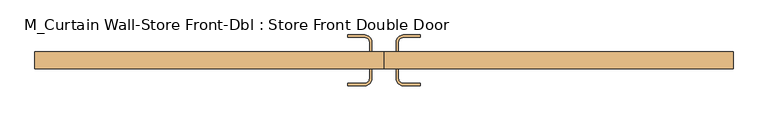
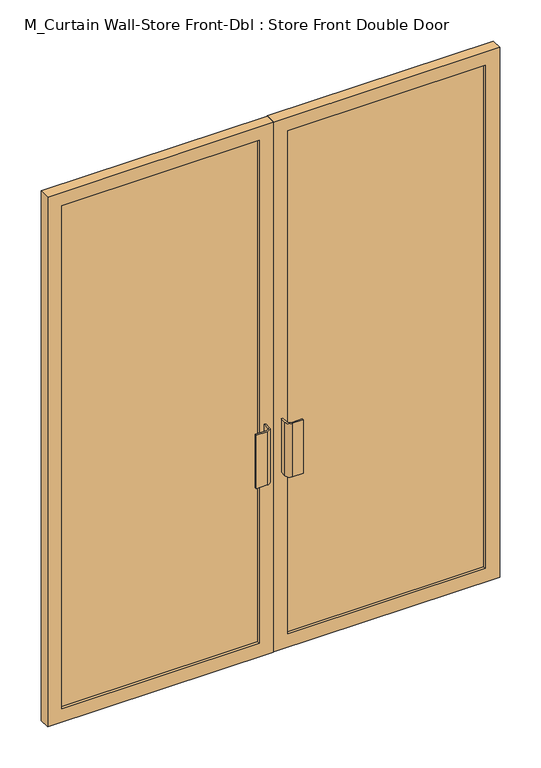
"""IFC4 building model written with IfcOpenShell, lengths in millimetres: door geometry, M_Curtain Wall-Store Front-Dbl : Store Front Double Door."""

from ifc_helpers import new_model, si_unit, point, frame, frame_2d, origin, place, context, project, spatial, polyline, circle_curve, trimmed, segment, composite_curve, outline, extrude, source, transform, mapped, element, save


def m_curtain_wall_store_front_dbl_store_front_double_door_46208f06(model_context):
    return source(origin(), model_context, "Body", "SweptSolid", [
        extrude(outline(composite_curve([segment(trimmed(circle_curve(frame_2d((-50.8, -14.85)), 19.05), [point((-31.75, -14.85))], [point((-50.8, -33.9))], False, "CARTESIAN"), True, "CONTINUOUS"), segment(polyline([(-50.8, -33.9), (-95.25, -33.9), (-95.25, -27.55), (-50.8, -27.55)]), True, "CONTINUOUS"), segment(trimmed(circle_curve(frame_2d((-50.8, -14.85)), 12.7), [point((-50.8, -27.55))], [point((-38.1, -14.85))], True, "CARTESIAN"), True, "CONTINUOUS"), segment(polyline([(-38.1, -14.85), (-38.1, 10.55), (-31.75, 10.55), (-31.75, -14.85)]), True, "CONTINUOUS")], self_intersect=False)), frame((0.0, 0.0, 762.0), z_axis=(0.0, 0.0, 1.0), x_axis=(1.0, 0.0, 0.0)), (0.0, 0.0, 1.0), 228.6),
        extrude(outline(composite_curve([segment(polyline([(31.75, -14.85), (31.75, 10.55), (38.1, 10.55), (38.1, -14.85)]), True, "CONTINUOUS"), segment(trimmed(circle_curve(frame_2d((50.8, -14.85)), 12.7), [point((38.1, -14.85))], [point((50.8, -27.55))], True, "CARTESIAN"), True, "CONTINUOUS"), segment(polyline([(50.8, -27.55), (95.25, -27.55), (95.25, -33.9), (50.8, -33.9)]), True, "CONTINUOUS"), segment(trimmed(circle_curve(frame_2d((50.8, -14.85)), 19.05), [point((50.8, -33.9))], [point((31.75, -14.85))], False, "CARTESIAN"), True, "CONTINUOUS")], self_intersect=False)), frame((0.0, 0.0, 762.0), z_axis=(0.0, 0.0, 1.0), x_axis=(1.0, 0.0, 0.0)), (0.0, 0.0, 1.0), 228.6),
        extrude(outline(composite_curve([segment(polyline([(-31.75, 80.4), (-31.75, 55.0), (-38.1, 55.0), (-38.1, 80.4)]), True, "CONTINUOUS"), segment(trimmed(circle_curve(frame_2d((-50.8, 80.4)), 12.7), [point((-38.1, 80.4))], [point((-50.8, 93.1))], True, "CARTESIAN"), True, "CONTINUOUS"), segment(polyline([(-50.8, 93.1), (-95.25, 93.1), (-95.25, 99.45), (-50.8, 99.45)]), True, "CONTINUOUS"), segment(trimmed(circle_curve(frame_2d((-50.8, 80.4)), 19.05), [point((-50.8, 99.45))], [point((-31.75, 80.4))], False, "CARTESIAN"), True, "CONTINUOUS")], self_intersect=False)), frame((0.0, 0.0, 762.0), z_axis=(0.0, 0.0, 1.0), x_axis=(1.0, 0.0, 0.0)), (0.0, 0.0, 1.0), 228.6),
        extrude(outline(composite_curve([segment(trimmed(circle_curve(frame_2d((50.8, 80.4)), 19.05), [point((31.75, 80.4))], [point((50.8, 99.45))], False, "CARTESIAN"), True, "CONTINUOUS"), segment(polyline([(50.8, 99.45), (95.25, 99.45), (95.25, 93.1), (50.8, 93.1)]), True, "CONTINUOUS"), segment(trimmed(circle_curve(frame_2d((50.8, 80.4)), 12.7), [point((50.8, 93.1))], [point((38.1, 80.4))], True, "CARTESIAN"), True, "CONTINUOUS"), segment(polyline([(38.1, 80.4), (38.1, 55.0), (31.75, 55.0), (31.75, 80.4)]), True, "CONTINUOUS")], self_intersect=False)), frame((0.0, 0.0, 762.0), z_axis=(0.0, 0.0, 1.0), x_axis=(1.0, 0.0, 0.0)), (0.0, 0.0, 1.0), 228.6),
        extrude(outline(polyline([(860.9333333, 23.25), (57.94375, 23.25), (57.94375, 42.3), (860.9333333, 42.3), (860.9333333, 23.25)])), frame((0.0, 0.0, 57.15), z_axis=(0.0, 0.0, 1.0), x_axis=(1.0, 0.0, 0.0)), (0.0, 0.0, 1.0), 2160.7),
        extrude(outline(polyline([(-57.94375, 23.25), (-860.9333333, 23.25), (-860.9333333, 42.3), (-57.94375, 42.3), (-57.94375, 23.25)])), frame((0.0, 0.0, 57.15), z_axis=(0.0, 0.0, 1.0), x_axis=(1.0, 0.0, 0.0)), (0.0, 0.0, 1.0), 2160.7),
        extrude(outline(polyline([(2275.0, 0.79375), (0.0, 0.79375), (0.0, 918.0833333), (2275.0, 918.0833333), (2275.0, 0.79375)]), holes=[polyline([(2217.85, 57.94375), (2217.85, 860.9333333), (57.15, 860.9333333), (57.15, 57.94375), (2217.85, 57.94375)])]), frame((0.0, 10.55, 0.0), z_axis=(0.0, 1.0, 0.0), x_axis=(0.0, 0.0, 1.0)), (0.0, 0.0, 1.0), 44.45),
        extrude(outline(polyline([(2275.0, -0.79375), (2275.0, -918.0833333), (0.0, -918.0833333), (0.0, -0.79375), (2275.0, -0.79375)]), holes=[polyline([(2217.85, -860.9333333), (2217.85, -57.94375), (57.15, -57.94375), (57.15, -860.9333333), (2217.85, -860.9333333)])]), frame((0.0, 10.55, 0.0), z_axis=(0.0, 1.0, 0.0), x_axis=(0.0, 0.0, 1.0)), (0.0, 0.0, 1.0), 44.45),
    ])


if __name__ == "__main__":
    model = new_model("IFC4")
    model_context = context("Model", 3, world=origin())
    ifc_project = project(units=[si_unit("LENGTHUNIT", "METRE", prefix="MILLI")], contexts=[model_context])
    site = spatial("IfcSite", under=ifc_project)
    building = spatial("IfcBuilding", under=site)
    placement = place(None, origin())
    m_curtain_wall_store_front_dbl_store_front_double_door_shape = m_curtain_wall_store_front_dbl_store_front_double_door_46208f06(model_context)
    element("IfcDoor", 1, ObjectType="M_Curtain Wall-Store Front-Dbl : Store Front Double Door", at=placement, inside=building, context=model_context, shape_type="MappedRepresentation", body=[
        mapped(m_curtain_wall_store_front_dbl_store_front_double_door_shape, transform((0.0, 0.0, 0.0), x_axis=(1.0, 0.0, 0.0), y_axis=(0.0, 1.0, 0.0), z_axis=(0.0, 0.0, 1.0))),
    ])
    save(model, "model.ifc")

# Revit data of these elements
# Type "M_Curtain Wall-Store Front-Dbl : Store Front Double Door"
#   Type Mark = "35"
#   Offset = 0.055 m
#   Function = 1
#   Define Thermal Properties by = 1
#   Material = Metal - Aluminum
#   Glazing Material = Window - Glass
#   Assembly Code = ""
# Element 1 (IfcDoor, "M_Curtain Wall-Store Front-Dbl : Store Front Double Door")
#   Materials on its faces: "Metal - Aluminum", "Window - Glass"
# Materials
#   "Metal - Aluminum": class "Unassigned", colour RGB 247 247 247, transparency 0, Comments = "Rendering appearance not upgraded "
#   "Window - Glass": class "Glas", colour RGB 128 128 255, transparency 0.75
